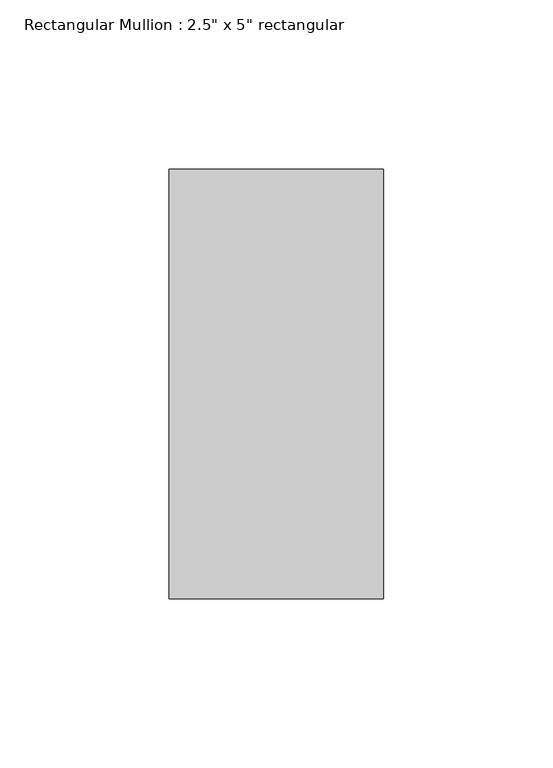
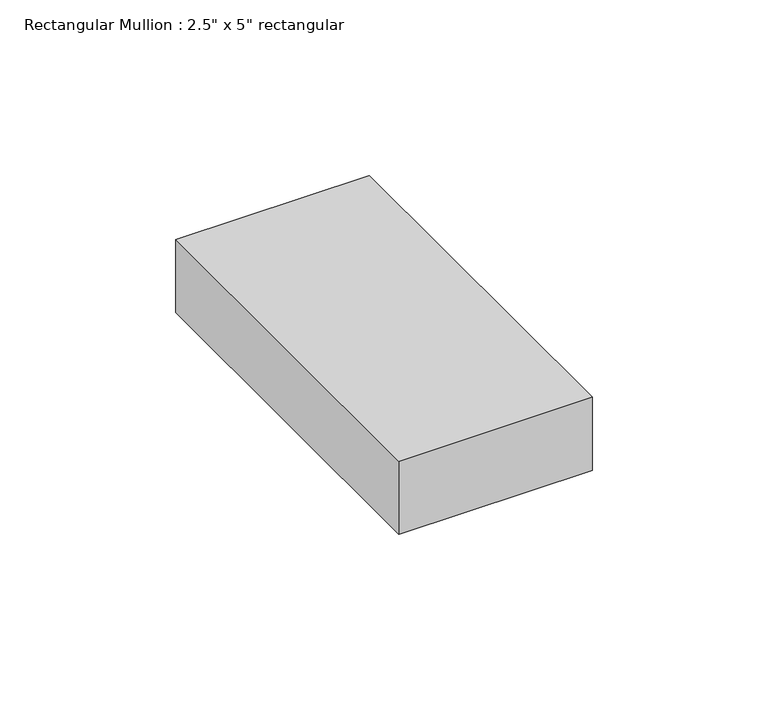
"""IFC4 building model written with IfcOpenShell, lengths in millimetres: member geometry."""

from ifc_helpers import new_model, si_unit, frame, origin, place, context, project, spatial, polyline, outline, extrude, source, transform, mapped, element, save


def member_0f16ceef(model_context):
    return source(origin(), model_context, "Body", "SweptSolid", [
        extrude(outline(polyline([(31.75, 63.5), (31.75, -63.5), (-31.75, -63.5), (-31.75, 63.5), (31.75, 63.5)])), frame((0.0, 0.0, -25.4), z_axis=(0.0, 0.0, 1.0), x_axis=(1.0, 0.0, 0.0)), (0.0, 0.0, 1.0), 25.4),
    ])


if __name__ == "__main__":
    model = new_model("IFC4")
    model_context = context("Model", 3, world=origin())
    ifc_project = project(units=[si_unit("LENGTHUNIT", "METRE", prefix="MILLI")], contexts=[model_context])
    site = spatial("IfcSite", under=ifc_project)
    building = spatial("IfcBuilding", under=site)
    placement = place(None, origin())
    member_shape = member_0f16ceef(model_context)
    element("IfcMember", 1, ObjectType="Rectangular Mullion : 2.5\" x 5\" rectangular", at=placement, inside=building, context=model_context, shape_type="MappedRepresentation", body=[
        mapped(member_shape, transform((0.0, 0.0, 0.0), x_axis=(1.0, 0.0, 0.0), y_axis=(0.0, 1.0, 0.0), z_axis=(0.0, 0.0, 1.0))),
    ])
    save(model, "model.ifc")

# Revit data of these elements
# Type "Rectangular Mullion : 2.5\" x 5\" rectangular"
#   built-in parameter 1007304 = 0.416667 (stored number, unit not read)
#   built-in parameter 1007301 = 0.104167 (stored number, unit not read)
#   built-in parameter 1007300 = 0.104167 (stored number, unit not read)
# Element 1 (IfcMember, "Rectangular Mullion : 2.5\" x 5\" rectangular")
#   Materials on its faces: "Metal - Aluminum"
# Materials
#   "Metal - Aluminum": class "Metal", colour RGB 140 140 140, transparency 0
